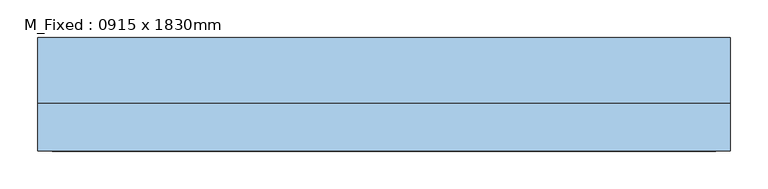
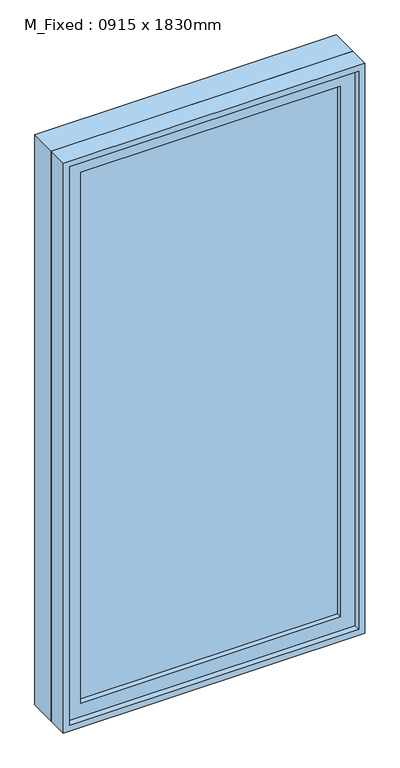
"""IFC4 building model written with IfcOpenShell, lengths in millimetres: window geometry, M_Fixed : 0915 x 1830mm."""

from ifc_helpers import new_model, si_unit, frame, origin, place, context, project, spatial, polyline, outline, extrude, source, transform, mapped, element, save


def m_fixed_0915_x_1830mm_6204a732(model_context):
    return source(origin(), model_context, "Body", "SweptSolid", [
        extrude(outline(polyline([(-394.5, -53.0), (-394.5, -41.0), (394.5, -41.0), (394.5, -53.0), (-394.5, -53.0)])), frame((0.0, 0.0, 368.0), z_axis=(0.0, 0.0, 1.0), x_axis=(1.0, 0.0, 0.0)), (0.0, 0.0, 1.0), 1704.0),
        extrude(outline(polyline([(2116.0, -438.5), (324.0, -438.5), (324.0, 438.5), (2116.0, 438.5), (2116.0, -438.5)]), holes=[polyline([(2072.0, -394.5), (2072.0, 394.5), (368.0, 394.5), (368.0, -394.5), (2072.0, -394.5)])]), frame((0.0, -69.0, 0.0), z_axis=(0.0, 1.0, 0.0), x_axis=(0.0, 0.0, 1.0)), (0.0, 0.0, 1.0), 44.0),
        extrude(outline(polyline([(2135.0, -457.5), (305.0, -457.5), (305.0, 457.5), (2135.0, 457.5), (2135.0, -457.5)]), holes=[polyline([(2116.0, -438.5), (2116.0, 438.5), (324.0, 438.5), (324.0, -438.5), (2116.0, -438.5)])]), frame((0.0, -88.0, 0.0), z_axis=(0.0, 1.0, 0.0), x_axis=(0.0, 0.0, 1.0)), (0.0, 0.0, 1.0), 63.0),
        extrude(outline(polyline([(2135.0, -457.5), (305.0, -457.5), (305.0, 457.5), (2135.0, 457.5), (2135.0, -457.5)]), holes=[polyline([(2103.0, -425.5), (2103.0, 425.5), (337.0, 425.5), (337.0, -425.5), (2103.0, -425.5)])]), frame((0.0, -25.0, 0.0), z_axis=(0.0, 1.0, 0.0), x_axis=(0.0, 0.0, 1.0)), (0.0, 0.0, 1.0), 87.0),
    ])


if __name__ == "__main__":
    model = new_model("IFC4")
    model_context = context("Model", 3, world=origin())
    ifc_project = project(units=[si_unit("LENGTHUNIT", "METRE", prefix="MILLI")], contexts=[model_context])
    site = spatial("IfcSite", under=ifc_project)
    building = spatial("IfcBuilding", under=site)
    placement = place(None, origin())
    m_fixed_0915_x_1830mm_shape = m_fixed_0915_x_1830mm_6204a732(model_context)
    element("IfcWindow", 1, ObjectType="M_Fixed : 0915 x 1830mm", at=placement, inside=building, context=model_context, shape_type="MappedRepresentation", body=[
        mapped(m_fixed_0915_x_1830mm_shape, transform((0.0, 0.0, 0.0), x_axis=(1.0, 0.0, 0.0), y_axis=(0.0, 1.0, 0.0), z_axis=(0.0, 0.0, 1.0))),
    ])
    save(model, "model.ifc")

# Revit data of these elements
# Type "M_Fixed : 0915 x 1830mm"
#   Type Mark = "18"
#   Height = 1.83 m
#   Default Sill Height = 0.305 m
#   Width = 0.915 m
#   Window Inset = 0.019 m
#   Frame Exterior Material = Sash
#   Frame Interior Material = Sash
#   Glass Pane Material = Glass
#   Sash = Sash
#   Wall Closure = (empty or 0)
# Element 1 (IfcWindow, "M_Fixed : 0915 x 1830mm")
#   Materials on its faces: "Sash", "Glass"
# Materials
#   "Sash": class "Wood", colour RGB 136 99 55, transparency 0
#   "Glass": class "Glass", colour RGB 247 249 248, transparency 0.85, Description = "Soda Lime Glass", Cost = 0
